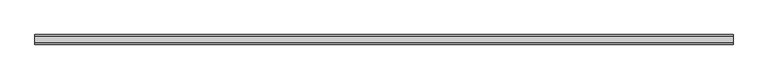
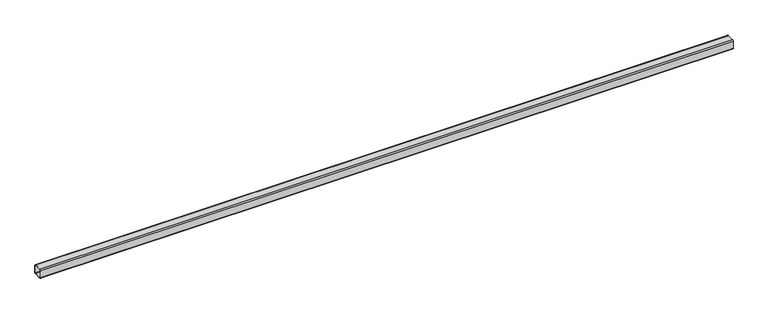
"""IFC4 building model written with IfcOpenShell, lengths in millimetres: beam geometry, Гнутый прямоугольный профиль (Трубы 30245-94) Балки : гнутый прямоуг. проф. 100x6."""

from ifc_helpers import new_model, si_unit, point, frame, frame_2d, origin, place, context, project, spatial, polyline, circle_curve, trimmed, segment, composite_curve, outline, extrude, source, transform, mapped, element, save


def beam_7f5963e0(model_context):
    return source(origin(), model_context, "Body", "SweptSolid", [
        extrude(outline(composite_curve([segment(polyline([(-38.0, 50.0), (38.0, 50.0)]), True, "CONTINUOUS"), segment(trimmed(circle_curve(frame_2d((38.0, 38.0)), 12.0), [point((38.0, 50.0))], [point((50.0, 38.0))], False, "CARTESIAN"), True, "CONTINUOUS"), segment(polyline([(50.0, 38.0), (50.0, -38.0)]), True, "CONTINUOUS"), segment(trimmed(circle_curve(frame_2d((38.0, -38.0)), 12.0), [point((50.0, -38.0))], [point((38.0, -50.0))], False, "CARTESIAN"), True, "CONTINUOUS"), segment(polyline([(38.0, -50.0), (-38.0, -50.0)]), True, "CONTINUOUS"), segment(trimmed(circle_curve(frame_2d((-38.0, -38.0)), 12.0), [point((-38.0, -50.0))], [point((-50.0, -38.0))], False, "CARTESIAN"), True, "CONTINUOUS"), segment(polyline([(-50.0, -38.0), (-50.0, 38.0)]), True, "CONTINUOUS"), segment(trimmed(circle_curve(frame_2d((-38.0, 38.0)), 12.0), [point((-50.0, 38.0))], [point((-38.0, 50.0))], False, "CARTESIAN"), True, "CONTINUOUS")], self_intersect=False), holes=[composite_curve([segment(trimmed(circle_curve(frame_2d((-38.0, 38.0)), 6.0), [point((-38.0, 44.0))], [point((-44.0, 38.0))], True, "CARTESIAN"), True, "CONTINUOUS"), segment(polyline([(-44.0, 38.0), (-44.0, -38.0)]), True, "CONTINUOUS"), segment(trimmed(circle_curve(frame_2d((-38.0, -38.0)), 6.0), [point((-44.0, -38.0))], [point((-38.0, -44.0))], True, "CARTESIAN"), True, "CONTINUOUS"), segment(polyline([(-38.0, -44.0), (38.0, -44.0)]), True, "CONTINUOUS"), segment(trimmed(circle_curve(frame_2d((38.0, -38.0)), 6.0), [point((38.0, -44.0))], [point((44.0, -38.0))], True, "CARTESIAN"), True, "CONTINUOUS"), segment(polyline([(44.0, -38.0), (44.0, 38.0)]), True, "CONTINUOUS"), segment(trimmed(circle_curve(frame_2d((38.0, 38.0)), 6.0), [point((44.0, 38.0))], [point((38.0, 44.0))], True, "CARTESIAN"), True, "CONTINUOUS"), segment(polyline([(38.0, 44.0), (-38.0, 44.0)]), True, "CONTINUOUS")], self_intersect=False)]), frame((-3634.0, 0.0, 0.0), z_axis=(1.0, 0.0, 0.0), x_axis=(0.0, 1.0, 0.0)), (0.0, 0.0, 1.0), 7268.0),
    ])


if __name__ == "__main__":
    model = new_model("IFC4")
    model_context = context("Model", 3, world=origin())
    ifc_project = project(units=[si_unit("LENGTHUNIT", "METRE", prefix="MILLI")], contexts=[model_context])
    site = spatial("IfcSite", under=ifc_project)
    building = spatial("IfcBuilding", under=site)
    placement = place(None, origin())
    beam_shape = beam_7f5963e0(model_context)
    element("IfcBeam", 1, ObjectType="Гнутый прямоугольный профиль (Трубы 30245-94) Балки : гнутый прямоуг. проф. 100x6", at=placement, inside=building, context=model_context, shape_type="MappedRepresentation", body=[
        mapped(beam_shape, transform((0.0, 0.0, 0.0), x_axis=(1.0, 0.0, 0.0), y_axis=(0.0, 1.0, 0.0), z_axis=(0.0, 0.0, 1.0))),
    ])
    save(model, "model.ifc")

# Revit data of these elements
# Type "Гнутый прямоугольный профиль (Трубы 30245-94) Балки : гнутый прямоуг. проф. 100x6"
#   ri = 12 mm
#   ra = 6 mm
#   W = 0.173578
#   Vz = 50 mm
#   Vy = 50 mm
#   Vpz = 50 mm
#   Vpy = 50 mm
#   Length [instance default] = 1500 mm
#   bf = 100 mm
#   d = 100 mm
#   tf = 6 mm
#   tw = 6 mm
#   A = 0.00226 m²
#   Structural Material [instance default] = Металл - Сталь - 345 МПa
#   Assembly Code = ""
# Element 1 (IfcBeam, "Гнутый прямоугольный профиль (Трубы 30245-94) Балки : гнутый прямоуг. проф. 100x6")
#   Structural Material = C235
#   Materials on its faces: "C235"
# Materials
#   "Металл - Сталь - 345 МПa": class "Металл", colour RGB 247 247 247, transparency 0
#   "C235": class "Не назначено", colour RGB 0 0 0, transparency 0
